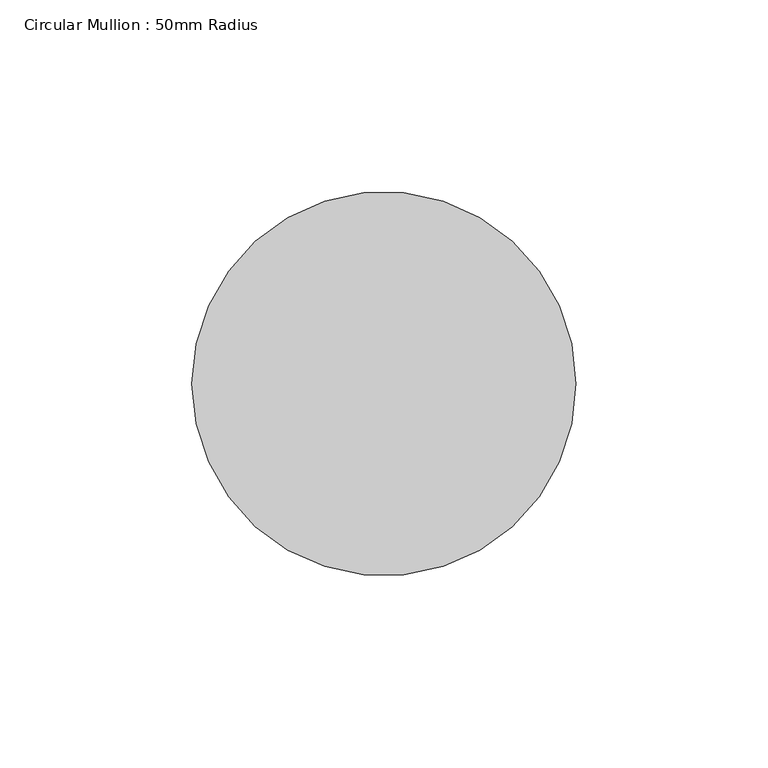
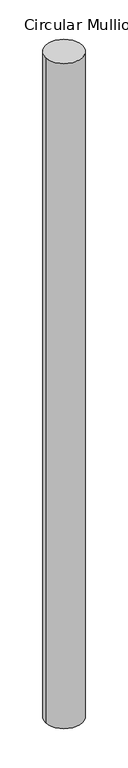
"""IFC4 building model written with IfcOpenShell, lengths in millimetres: member geometry, Circular Mullion : 50mm Radius."""

from ifc_helpers import new_model, si_unit, point, frame, frame_2d, origin, place, context, project, spatial, circle_curve, trimmed, segment, composite_curve, outline, extrude, source, transform, mapped, element, save


def circular_mullion_50mm_radius_ec3ba2f5(model_context):
    return source(origin(), model_context, "Body", "SweptSolid", [
        extrude(outline(composite_curve([segment(trimmed(circle_curve(frame_2d((-50.0, 0.0)), 50.0), [point((0.0, 0.0))], [point((-100.0, 0.0))], False, "CARTESIAN"), True, "CONTINUOUS"), segment(trimmed(circle_curve(frame_2d((-50.0, 0.0)), 50.0), [point((-100.0, 0.0))], [point((0.0, 0.0))], False, "CARTESIAN"), True, "CONTINUOUS")], self_intersect=False)), frame((0.0, 0.0, -1910.9246852), z_axis=(0.0, 0.0, 1.0), x_axis=(1.0, 0.0, 0.0)), (0.0, 0.0, 1.0), 1910.9246852),
    ])


if __name__ == "__main__":
    model = new_model("IFC4")
    model_context = context("Model", 3, world=origin())
    ifc_project = project(units=[si_unit("LENGTHUNIT", "METRE", prefix="MILLI")], contexts=[model_context])
    site = spatial("IfcSite", under=ifc_project)
    building = spatial("IfcBuilding", under=site)
    placement = place(None, origin())
    circular_mullion_50mm_radius_shape = circular_mullion_50mm_radius_ec3ba2f5(model_context)
    element("IfcMember", 1, ObjectType="Circular Mullion : 50mm Radius", at=placement, inside=building, context=model_context, shape_type="MappedRepresentation", body=[
        mapped(circular_mullion_50mm_radius_shape, transform((0.0, 0.0, 0.0), x_axis=(1.0, 0.0, 0.0), y_axis=(0.0, 1.0, 0.0), z_axis=(0.0, 0.0, 1.0))),
    ])
    save(model, "model.ifc")

# Revit data of these elements
# Type "Circular Mullion : 50mm Radius"
#   built-in parameter 1007350 = 0.164042 (stored number, unit not read)
# Element 1 (IfcMember, "Circular Mullion : 50mm Radius")
#   Materials on its faces: "Aluminium"
# Materials
#   "Aluminium": class "Metal", colour RGB 247 247 247, transparency 0, Description = "Aluminium 6061", Cost = 0
